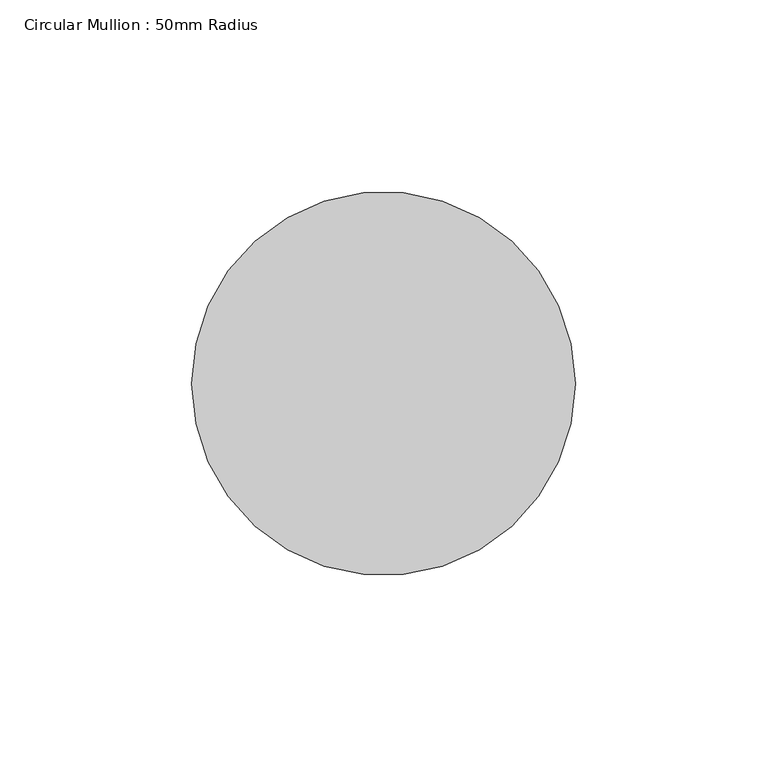
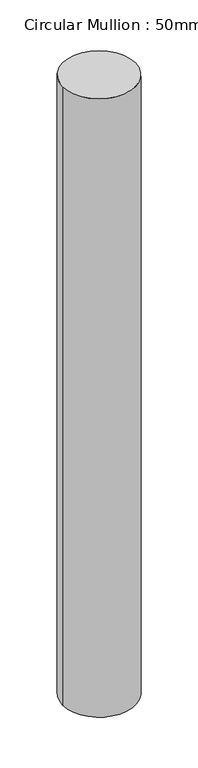
"""IFC4 building model written with IfcOpenShell, lengths in millimetres: member geometry, Circular Mullion : 50mm Radius."""

from ifc_helpers import new_model, si_unit, point, frame, origin, origin_2d, place, context, project, spatial, circle_curve, trimmed, segment, composite_curve, outline, extrude, source, transform, mapped, element, save


def circular_mullion_50mm_radius_0e846bcb(model_context):
    return source(origin(), model_context, "Body", "SweptSolid", [
        extrude(outline(composite_curve([segment(trimmed(circle_curve(origin_2d(), 50.0), [point((50.0, 0.0))], [point((-50.0, 0.0))], False, "CARTESIAN"), True, "CONTINUOUS"), segment(trimmed(circle_curve(origin_2d(), 50.0), [point((-50.0, 0.0))], [point((50.0, 0.0))], False, "CARTESIAN"), True, "CONTINUOUS")], self_intersect=False)), frame((0.0, 0.0, -899.7984549), z_axis=(0.0, 0.0, 1.0), x_axis=(1.0, 0.0, 0.0)), (0.0, 0.0, 1.0), 899.7984549),
    ])


if __name__ == "__main__":
    model = new_model("IFC4")
    model_context = context("Model", 3, world=origin())
    ifc_project = project(units=[si_unit("LENGTHUNIT", "METRE", prefix="MILLI")], contexts=[model_context])
    site = spatial("IfcSite", under=ifc_project)
    building = spatial("IfcBuilding", under=site)
    placement = place(None, origin())
    circular_mullion_50mm_radius_shape = circular_mullion_50mm_radius_0e846bcb(model_context)
    element("IfcMember", 1, ObjectType="Circular Mullion : 50mm Radius", at=placement, inside=building, context=model_context, shape_type="MappedRepresentation", body=[
        mapped(circular_mullion_50mm_radius_shape, transform((0.0, 0.0, 0.0), x_axis=(1.0, 0.0, 0.0), y_axis=(0.0, 1.0, 0.0), z_axis=(0.0, 0.0, 1.0))),
    ])
    save(model, "model.ifc")

# Revit data of these elements
# Type "Circular Mullion : 50mm Radius"
#   built-in parameter 1007350 = 0.164042 (stored number, unit not read)
# Element 1 (IfcMember, "Circular Mullion : 50mm Radius")
#   Materials on its faces: "Aluminium"
# Materials
#   "Aluminium": class "Metal", colour RGB 247 247 247, transparency 0, Description = "Aluminium 6061", Cost = 0
